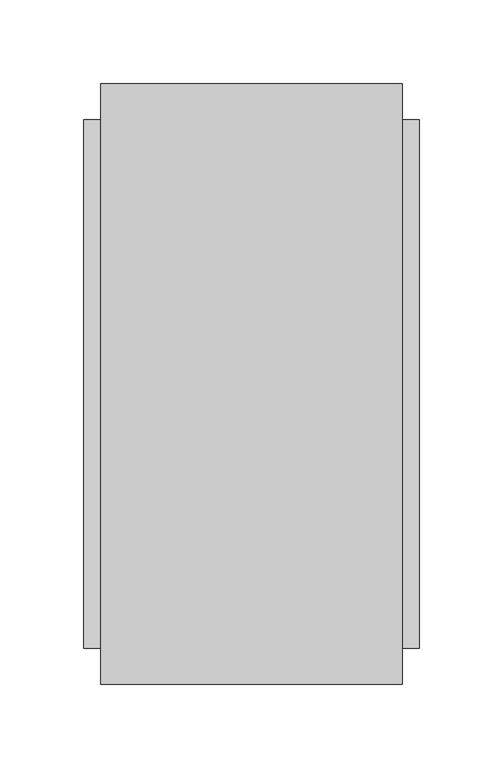
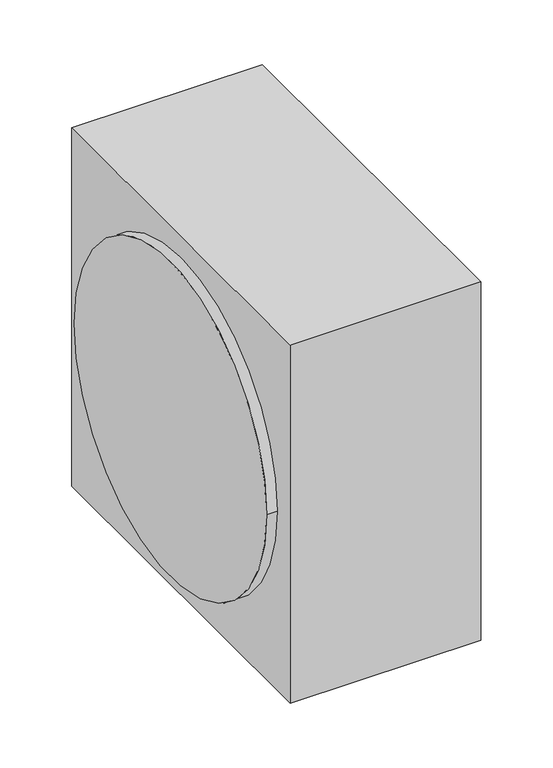
"""IFC4 building model written with IfcOpenShell, lengths in millimetres: proxy geometry, Фильтр кассетный DRF : Фильтр кассетный DRF 315."""

from ifc_helpers import new_model, si_unit, point, frame, origin, origin_2d, place, context, project, spatial, polyline, circle_curve, trimmed, segment, composite_curve, outline, extrude, source, transform, mapped, element, save


def mechanical_equipment_2655a0ad(model_context):
    return source(origin(), model_context, "Body", "SweptSolid", [
        extrude(outline(composite_curve([segment(trimmed(circle_curve(origin_2d(), 157.5), [point((-157.5, 0.0))], [point((157.5, 0.0))], False, "CARTESIAN"), True, "CONTINUOUS"), segment(trimmed(circle_curve(origin_2d(), 157.5), [point((157.5, 0.0))], [point((-157.5, 0.0))], False, "CARTESIAN"), True, "CONTINUOUS")], self_intersect=False)), frame((-100.0, 0.0, 0.0), z_axis=(1.0, 0.0, 0.0), x_axis=(0.0, 1.0, 0.0)), (0.0, 0.0, 1.0), 10.0),
        extrude(outline(composite_curve([segment(trimmed(circle_curve(origin_2d(), 157.5), [point((-157.5, 0.0))], [point((157.5, 0.0))], False, "CARTESIAN"), True, "CONTINUOUS"), segment(trimmed(circle_curve(origin_2d(), 157.5), [point((157.5, 0.0))], [point((-157.5, 0.0))], False, "CARTESIAN"), True, "CONTINUOUS")], self_intersect=False)), frame((90.0, 0.0, 0.0), z_axis=(1.0, 0.0, 0.0), x_axis=(0.0, 1.0, 0.0)), (0.0, 0.0, 1.0), 10.0),
        extrude(outline(polyline([(90.0, 179.0), (90.0, -179.0), (-90.0, -179.0), (-90.0, 179.0), (90.0, 179.0)])), frame((0.0, 0.0, -179.0), z_axis=(0.0, 0.0, 1.0), x_axis=(1.0, 0.0, 0.0)), (0.0, 0.0, 1.0), 358.0),
    ])


if __name__ == "__main__":
    model = new_model("IFC4")
    model_context = context("Model", 3, world=origin())
    ifc_project = project(units=[si_unit("LENGTHUNIT", "METRE", prefix="MILLI")], contexts=[model_context])
    site = spatial("IfcSite", under=ifc_project)
    building = spatial("IfcBuilding", under=site)
    placement = place(None, origin())
    mechanical_equipment_shape = mechanical_equipment_2655a0ad(model_context)
    element("IfcBuildingElementProxy", 1, Name="Фильтр кассетный DRF : Фильтр кассетный DRF 315", ObjectType="Фильтр кассетный DRF : Фильтр кассетный DRF 315", at=placement, inside=building, context=model_context, shape_type="MappedRepresentation", body=[
        mapped(mechanical_equipment_shape, transform((0.0, 0.0, 0.0), x_axis=(1.0, 0.0, 0.0), y_axis=(0.0, 1.0, 0.0), z_axis=(0.0, 0.0, 1.0))),
    ])
    save(model, "model.ifc")

# Revit data of these elements
# Project information
#   Название организации = "Название организации"
#   Описание организации = "Описание организации"
#   Наименование здания = "Наименование здания"
#   Заказчик = "Заказчик"
#   Адрес проекта = "Адрес проекта"
#   Наименование проекта = "Наименование проекта"
# Type "Фильтр кассетный DRF : Фильтр кассетный DRF 315"
#   ADSK_Система_Имя [instance default] = ""
#   ADSK_Наименование краткое = "DRF 315"
#   ADSK_Наименование [instance default] = "Фильтр кассетный DRF 315"
#   ADSK_Масса_Текст = "13.29"
#   ADSK_Марка = ""
#   ADSK_Код изделия = ""
#   ADSK_Завод-изготовитель = "WAER"
#   ADSK_Единица измерения = "шт."
#   ADSK_URL страницы изделия = ""
#   ADSK_URL документации изделия = ""
#   ADSK_Расход воздуха = 0 m³/h
#   ADSK_Размер_Ширина_H = 358 mm
#   ADSK_Размер_Диаметр_D = 315 mm
#   ADSK_Потеря давления воздуха = 0.0 Pa
#   ADSK_Масса = 13.29
#   ADSK_Количество [instance default] = 1
#   Default Elevation = 0
#   URL = ""
#   Cost = 0
